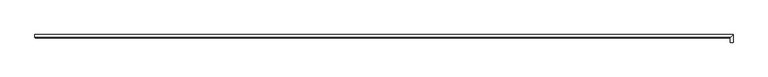
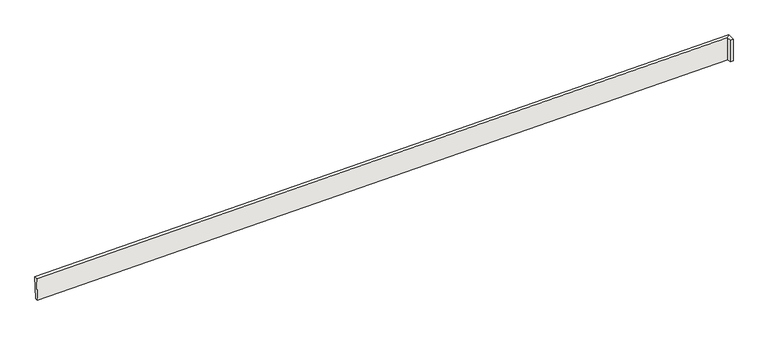
"""IFC4 building model written with IfcOpenShell, lengths in millimetres: slab geometry, FECHAMENTO DECK MADEIRA - RAMPA ENTRADA1 : CC_ND 300 FECHAMENTO 2 x 15 cm DECK MADEIRA - RAMPA ENTRADA."""

import ifcopenshell
import ifcopenshell.guid

model = None  # the IFC model being written
_history = None  # IfcOwnerHistory: only IFC2X3 demands one
_inside = {}  # id of a spatial element -> (the spatial element, [elements in it])
_under = {}  # id of a project, library or spatial element -> (it, [spatial elements below it])
_declared = {}  # id of a project -> (the project, [libraries it declares])
_typed = {}  # id of a type object -> (the type object, [elements of that type])
_made_of = {}  # id of a material, layer set ... -> (it, [elements and type objects made of it])


def new_model(schema):
    """Start an empty IFC model of exactly this schema.

    Asked for "IFC4X3", IfcOpenShell would pick the latest addendum, in which some entities
    have other attributes; the version numbers below select the first issue.
    IFC2X3 requires an IfcOwnerHistory on every rooted entity: one is made here for all.
    """
    global model, _history
    if schema == "IFC4X3":
        model = ifcopenshell.file(schema_version=(4, 3, 0, 0))
    else:
        model = ifcopenshell.file(schema=schema)
    _inside.clear()
    _under.clear()
    _declared.clear()
    _typed.clear()
    _made_of.clear()
    _history = None
    if model.schema == "IFC2X3":
        org = make("IfcOrganization", Name="unknown")
        user = make(
            "IfcPersonAndOrganization",
            ThePerson=make("IfcPerson", FamilyName="unknown"),
            TheOrganization=org,
        )
        app = make(
            "IfcApplication",
            ApplicationDeveloper=org,
            Version="unknown",
            ApplicationFullName="unknown",
            ApplicationIdentifier="unknown",
        )
        _history = make(
            "IfcOwnerHistory",
            OwningUser=user,
            OwningApplication=app,
            ChangeAction="ADDED",
            CreationDate=0,
        )
    return model


def make(cls, **values):
    """One entity of the class cls with the attributes given. An attribute that is None is left unset."""
    return model.create_entity(
        cls, **{name: value for name, value in values.items() if value is not None}
    )


def rooted(cls, **values):
    """An entity with a GlobalId (a new one), such as an element, a storey or a relation."""
    return make(cls, GlobalId=ifcopenshell.guid.new(), OwnerHistory=_history, **values)


def si_unit(unit_type, name, prefix=None):
    """IfcSIUnit, for example si_unit("LENGTHUNIT", "METRE", prefix="MILLI")."""
    return make("IfcSIUnit", UnitType=unit_type, Prefix=prefix, Name=name)


def assignment(units):
    """IfcUnitAssignment: the units of a project."""
    return None if units is None else make("IfcUnitAssignment", Units=units)


def point(xyz):
    """IfcCartesianPoint."""
    return None if xyz is None else make("IfcCartesianPoint", Coordinates=xyz)


def direction(xyz):
    """IfcDirection."""
    return None if xyz is None else make("IfcDirection", DirectionRatios=xyz)


def frame(location, z_axis=None, x_axis=None):
    """IfcAxis2Placement3D, a coordinate frame: its origin and axes. An axis left out is left unset."""
    return make(
        "IfcAxis2Placement3D",
        Location=point(location),
        Axis=direction(z_axis),
        RefDirection=direction(x_axis),
    )


def origin():
    """The frame at (0, 0, 0) with its axes left unset."""
    return frame((0.0, 0.0, 0.0))


def place(relative_to, where):
    """IfcLocalPlacement: puts the frame where relative to a parent placement (None: the world)."""
    return make(
        "IfcLocalPlacement", PlacementRelTo=relative_to, RelativePlacement=where
    )


def context(
    kind, dimensions, precision=None, world=None, true_north=None, identifier=None
):
    """IfcGeometricRepresentationContext, for example the 3D "Model" context."""
    return make(
        "IfcGeometricRepresentationContext",
        ContextIdentifier=identifier,
        ContextType=kind,
        CoordinateSpaceDimension=dimensions,
        Precision=precision,
        WorldCoordinateSystem=world,
        TrueNorth=true_north,
    )


def project(units=None, contexts=None):
    """IfcProject with its units and contexts."""
    return rooted(
        "IfcProject",
        Name="project",
        RepresentationContexts=contexts,
        UnitsInContext=assignment(units),
    )


def spatial(cls, under=None, at=None, **own):
    """A site, building, storey or space (cls), placed at a placement, below another one or the project."""
    s = rooted(cls, ObjectPlacement=at, **own)
    if under is not None:
        _under.setdefault(under.id(), (under, []))[1].append(s)
    return s


def faces_of(points, faces, orient=None, outer=None):
    """IfcFace entities. A face is a list of loops; a loop is a list of indices into points, from 0.

    orient and outer hold one flag for each loop. By default every Orientation is true, the
    first loop of a face is its IfcFaceOuterBound and the others are IfcFaceBound.
    """
    made = []
    for i, loops in enumerate(faces):
        bounds = []
        for j, loop in enumerate(loops):
            is_outer = j == 0 if outer is None else outer[i][j]
            bounds.append(
                make(
                    "IfcFaceOuterBound" if is_outer else "IfcFaceBound",
                    Bound=make("IfcPolyLoop", Polygon=[points[k] for k in loop]),
                    Orientation=True if orient is None else orient[i][j],
                )
            )
        made.append(make("IfcFace", Bounds=bounds))
    return made


def faceted_brep(points, faces, orient=None, outer=None, voids=None):
    """IfcFacetedBrep: a solid bounded by flat faces; with voids (closed shells), ...WithVoids."""
    shared = [point(p) for p in points]
    hull = make("IfcClosedShell", CfsFaces=faces_of(shared, faces, orient, outer))
    if voids is None:
        return make("IfcFacetedBrep", Outer=hull)
    return make(
        "IfcFacetedBrepWithVoids",
        Outer=hull,
        Voids=[
            make(cls, CfsFaces=faces_of(shared, fs, o, b)) for cls, fs, o, b in voids
        ],
    )


def shape(context_of_items, identifier, shape_type, items):
    """IfcShapeRepresentation: the items that make up one representation, for example the "Body"."""
    return make(
        "IfcShapeRepresentation",
        ContextOfItems=context_of_items,
        RepresentationIdentifier=identifier,
        RepresentationType=shape_type,
        Items=items,
    )


def source(mapping_origin, context_of_items, identifier, shape_type, items):
    """IfcRepresentationMap: a shape defined once, which mapped items show again and again."""
    return make(
        "IfcRepresentationMap",
        MappingOrigin=mapping_origin,
        MappedRepresentation=shape(context_of_items, identifier, shape_type, items),
    )


def transform(
    local_origin,
    x_axis=None,
    y_axis=None,
    z_axis=None,
    scale=None,
    scale2=None,
    scale3=None,
    uniform=True,
):
    """IfcCartesianTransformationOperator3D, or its non-uniform kind. x_axis, y_axis, z_axis: its Axis1, 2, 3."""
    if uniform:
        return make(
            "IfcCartesianTransformationOperator3D",
            Axis1=direction(x_axis),
            Axis2=direction(y_axis),
            LocalOrigin=point(local_origin),
            Scale=scale,
            Axis3=direction(z_axis),
        )
    return make(
        "IfcCartesianTransformationOperator3DnonUniform",
        Axis1=direction(x_axis),
        Axis2=direction(y_axis),
        LocalOrigin=point(local_origin),
        Scale=scale,
        Axis3=direction(z_axis),
        Scale2=scale2,
        Scale3=scale3,
    )


def mapped(mapping_source, mapping_target):
    """IfcMappedItem: shows the shape of a source again, moved by a transform."""
    return make(
        "IfcMappedItem", MappingSource=mapping_source, MappingTarget=mapping_target
    )


def made_of(thing, what):
    """Note that an element or type object is made of a material, layer set ...; save() writes the relation."""
    if what is not None:
        _made_of.setdefault(what.id(), (what, []))[1].append(thing)
    return thing


def element(
    cls,
    number,
    at=None,
    inside=None,
    cuts=None,
    type_object=None,
    material=None,
    context=None,
    identifier="Body",
    shape_type=None,
    held_by="IfcProductDefinitionShape",
    body=None,
    shapes=None,
    **own,
):
    """One element of the class cls, such as IfcWall. Its Tag is "e" and its number.

    at: its placement. inside: the storey or other place that contains it. cuts: it is an
    opening in that element (IfcRelVoidsElement). A single representation is given by context,
    identifier, shape_type and body (its items); several are given by shapes. held_by: the class
    of the entity that holds the representations. save() writes the other relations.
    """
    e = rooted(cls, Tag="e%d" % number, ObjectPlacement=at, **own)
    if body is not None:
        shapes = [shape(context, identifier, shape_type, body)]
    if shapes is not None:
        e.Representation = make(held_by, Representations=shapes)
    if inside is not None:
        _inside.setdefault(inside.id(), (inside, []))[1].append(e)
    if cuts is not None:
        rooted(
            "IfcRelVoidsElement", RelatingBuildingElement=cuts, RelatedOpeningElement=e
        )
    if type_object is not None:
        _typed.setdefault(type_object.id(), (type_object, []))[1].append(e)
    return made_of(e, material)


def aggregate(whole, parts):
    """IfcRelAggregates: a whole, such as a stair, and the parts it consists of."""
    return rooted("IfcRelAggregates", RelatingObject=whole, RelatedObjects=parts)


def save(model, path):
    """Write the relations noted so far, then the file.

    IfcRelAggregates (storeys below a building ...), IfcRelContainedInSpatialStructure (elements
    in a storey), IfcRelDefinesByType, IfcRelAssociatesMaterial and IfcRelDeclares: one each for
    every whole, place, type object, material and project.
    """
    for whole, parts in _under.values():
        aggregate(whole, parts)
    for where, things in _inside.values():
        rooted(
            "IfcRelContainedInSpatialStructure",
            RelatedElements=things,
            RelatingStructure=where,
        )
    for kind, things in _typed.values():
        rooted("IfcRelDefinesByType", RelatedObjects=things, RelatingType=kind)
    for what, things in _made_of.values():
        rooted("IfcRelAssociatesMaterial", RelatedObjects=things, RelatingMaterial=what)
    for by, libraries in _declared.values():
        rooted("IfcRelDeclares", RelatingContext=by, RelatedDefinitions=libraries)
    model.write(path)


def slab_f1ba5172(model_context):
    return source(origin(), model_context, "Body", "Brep", [
        faceted_brep([(-16956.4780242, -1998.3737573, -69.9475924), (-16956.4850119, -2018.3702631, -69.5738214), (-16959.2882946, -2015.5664906, 80.373771), (-16959.281307, -1995.5699847, 80.0), (-12410.281307, -1998.3737573, 15.0439334), (-12430.281307, -2018.3702631, 15.0439334), (-12430.281307, -2015.5664906, 165.0439334), (-12410.281307, -1995.5699847, 165.0439334), (-12410.281307, -2045.5699847, 15.0439334), (-12410.281307, -2045.5699847, 165.0439334), (-12430.281307, -2045.5699847, 165.0439334), (-12430.281307, -2045.5699847, 15.0439334)], [[[0, 1, 2, 3]], [[1, 0, 4, 5]], [[2, 1, 5, 6]], [[3, 2, 6, 7]], [[0, 3, 7, 4]], [[8, 9, 10, 11]], [[5, 4, 8, 11]], [[6, 5, 11, 10]], [[7, 6, 10, 9]], [[4, 7, 9, 8]]]),
    ])


if __name__ == "__main__":
    model = new_model("IFC4")
    model_context = context("Model", 3, world=origin())
    ifc_project = project(units=[si_unit("LENGTHUNIT", "METRE", prefix="MILLI")], contexts=[model_context])
    site = spatial("IfcSite", under=ifc_project)
    building = spatial("IfcBuilding", under=site)
    placement = place(None, origin())
    slab_shape = slab_f1ba5172(model_context)
    element("IfcSlab", 1, ObjectType="FECHAMENTO DECK MADEIRA - RAMPA ENTRADA1 : CC_ND 300 FECHAMENTO 2 x 15 cm DECK MADEIRA - RAMPA ENTRADA", at=placement, inside=building, context=model_context, shape_type="MappedRepresentation", body=[
        mapped(slab_shape, transform((0.0, 0.0, 0.0), x_axis=(1.0, 0.0, 0.0), y_axis=(0.0, 1.0, 0.0), z_axis=(0.0, 0.0, 1.0))),
    ])
    save(model, "model.ifc")

# Revit data of these elements
# Type "FECHAMENTO DECK MADEIRA - RAMPA ENTRADA1 : CC_ND 300 FECHAMENTO 2 x 15 cm DECK MADEIRA - RAMPA ENTRADA"
#   Structural Material = .DECK DE MADEIRA LONGITUDINAL
# Element 1 (IfcSlab, "FECHAMENTO DECK MADEIRA - RAMPA ENTRADA1 : CC_ND 300 FECHAMENTO 2 x 15 cm DECK MADEIRA - RAMPA ENTRADA")
#   Materials on its faces: ".DECK DE MADEIRA LONGITUDINAL"
# Materials
#   ".DECK DE MADEIRA LONGITUDINAL": class ".CC_MADEIRA REVEST.", colour RGB 169 114 85, transparency 0, Description = "Deck de madeira", Cost = 0
